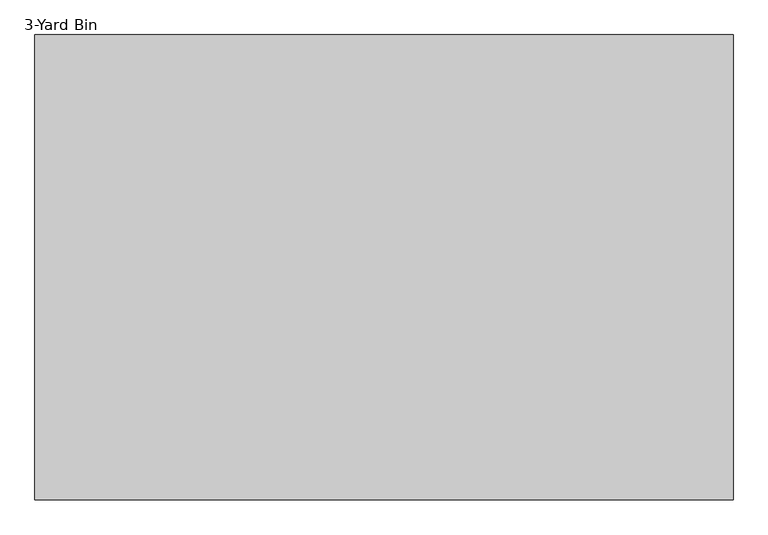
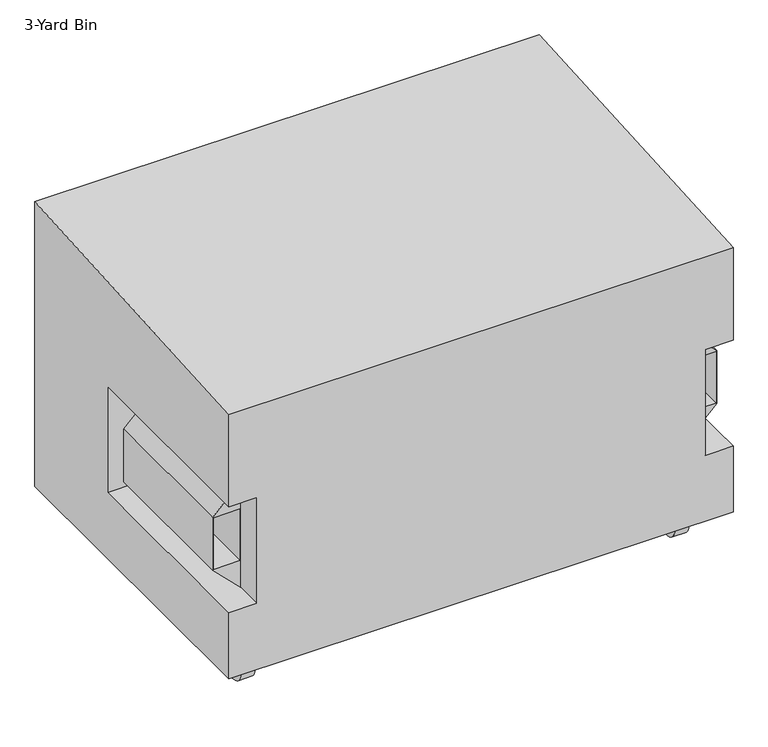
"""IFC4 building model written with IfcOpenShell, lengths in millimetres: proxy geometry, 323323 - Site Trash and Litter Receptacles - Dumpsters : 3-Yard Bin."""

import ifcopenshell
import ifcopenshell.guid

model = None  # the IFC model being written
_history = None  # IfcOwnerHistory: only IFC2X3 demands one
_inside = {}  # id of a spatial element -> (the spatial element, [elements in it])
_under = {}  # id of a project, library or spatial element -> (it, [spatial elements below it])
_declared = {}  # id of a project -> (the project, [libraries it declares])
_typed = {}  # id of a type object -> (the type object, [elements of that type])
_made_of = {}  # id of a material, layer set ... -> (it, [elements and type objects made of it])


def new_model(schema):
    """Start an empty IFC model of exactly this schema.

    Asked for "IFC4X3", IfcOpenShell would pick the latest addendum, in which some entities
    have other attributes; the version numbers below select the first issue.
    IFC2X3 requires an IfcOwnerHistory on every rooted entity: one is made here for all.
    """
    global model, _history
    if schema == "IFC4X3":
        model = ifcopenshell.file(schema_version=(4, 3, 0, 0))
    else:
        model = ifcopenshell.file(schema=schema)
    _inside.clear()
    _under.clear()
    _declared.clear()
    _typed.clear()
    _made_of.clear()
    _history = None
    if model.schema == "IFC2X3":
        org = make("IfcOrganization", Name="unknown")
        user = make(
            "IfcPersonAndOrganization",
            ThePerson=make("IfcPerson", FamilyName="unknown"),
            TheOrganization=org,
        )
        app = make(
            "IfcApplication",
            ApplicationDeveloper=org,
            Version="unknown",
            ApplicationFullName="unknown",
            ApplicationIdentifier="unknown",
        )
        _history = make(
            "IfcOwnerHistory",
            OwningUser=user,
            OwningApplication=app,
            ChangeAction="ADDED",
            CreationDate=0,
        )
    return model


def make(cls, **values):
    """One entity of the class cls with the attributes given. An attribute that is None is left unset."""
    return model.create_entity(
        cls, **{name: value for name, value in values.items() if value is not None}
    )


def rooted(cls, **values):
    """An entity with a GlobalId (a new one), such as an element, a storey or a relation."""
    return make(cls, GlobalId=ifcopenshell.guid.new(), OwnerHistory=_history, **values)


def si_unit(unit_type, name, prefix=None):
    """IfcSIUnit, for example si_unit("LENGTHUNIT", "METRE", prefix="MILLI")."""
    return make("IfcSIUnit", UnitType=unit_type, Prefix=prefix, Name=name)


def assignment(units):
    """IfcUnitAssignment: the units of a project."""
    return None if units is None else make("IfcUnitAssignment", Units=units)


def point(xyz):
    """IfcCartesianPoint."""
    return None if xyz is None else make("IfcCartesianPoint", Coordinates=xyz)


def direction(xyz):
    """IfcDirection."""
    return None if xyz is None else make("IfcDirection", DirectionRatios=xyz)


def frame(location, z_axis=None, x_axis=None):
    """IfcAxis2Placement3D, a coordinate frame: its origin and axes. An axis left out is left unset."""
    return make(
        "IfcAxis2Placement3D",
        Location=point(location),
        Axis=direction(z_axis),
        RefDirection=direction(x_axis),
    )


def frame_2d(location, x_axis=None):
    """IfcAxis2Placement2D, a coordinate frame in the plane: its origin and x axis."""
    return make(
        "IfcAxis2Placement2D", Location=point(location), RefDirection=direction(x_axis)
    )


def origin():
    """The frame at (0, 0, 0) with its axes left unset."""
    return frame((0.0, 0.0, 0.0))


def place(relative_to, where):
    """IfcLocalPlacement: puts the frame where relative to a parent placement (None: the world)."""
    return make(
        "IfcLocalPlacement", PlacementRelTo=relative_to, RelativePlacement=where
    )


def context(
    kind, dimensions, precision=None, world=None, true_north=None, identifier=None
):
    """IfcGeometricRepresentationContext, for example the 3D "Model" context."""
    return make(
        "IfcGeometricRepresentationContext",
        ContextIdentifier=identifier,
        ContextType=kind,
        CoordinateSpaceDimension=dimensions,
        Precision=precision,
        WorldCoordinateSystem=world,
        TrueNorth=true_north,
    )


def project(units=None, contexts=None):
    """IfcProject with its units and contexts."""
    return rooted(
        "IfcProject",
        Name="project",
        RepresentationContexts=contexts,
        UnitsInContext=assignment(units),
    )


def spatial(cls, under=None, at=None, **own):
    """A site, building, storey or space (cls), placed at a placement, below another one or the project."""
    s = rooted(cls, ObjectPlacement=at, **own)
    if under is not None:
        _under.setdefault(under.id(), (under, []))[1].append(s)
    return s


def circle_curve(where, radius):
    """IfcCircle in the frame where."""
    return make("IfcCircle", Position=where, Radius=radius)


def trimmed(basis, trim1, trim2, sense, master):
    """IfcTrimmedCurve: the piece of a basis curve between two trims."""
    return make(
        "IfcTrimmedCurve",
        BasisCurve=basis,
        Trim1=trim1,
        Trim2=trim2,
        SenseAgreement=sense,
        MasterRepresentation=master,
    )


def segment(curve, same_sense, transition):
    """IfcCompositeCurveSegment."""
    return make(
        "IfcCompositeCurveSegment",
        Transition=transition,
        SameSense=same_sense,
        ParentCurve=curve,
    )


def composite_curve(segments, self_intersect=None):
    """IfcCompositeCurve: segments joined end to end."""
    return make("IfcCompositeCurve", Segments=segments, SelfIntersect=self_intersect)


def outline(outer, holes=None, kind="AREA"):
    """IfcArbitraryClosedProfileDef: a profile drawn as a closed curve; with holes, ...WithVoids."""
    if holes is None:
        return make("IfcArbitraryClosedProfileDef", ProfileType=kind, OuterCurve=outer)
    return make(
        "IfcArbitraryProfileDefWithVoids",
        ProfileType=kind,
        OuterCurve=outer,
        InnerCurves=holes,
    )


def extrude(swept, where, along, depth):
    """IfcExtrudedAreaSolid: the profile swept, set in the frame where, extruded along a direction by depth."""
    return make(
        "IfcExtrudedAreaSolid",
        SweptArea=swept,
        Position=where,
        ExtrudedDirection=direction(along),
        Depth=depth,
    )


def faces_of(points, faces, orient=None, outer=None):
    """IfcFace entities. A face is a list of loops; a loop is a list of indices into points, from 0.

    orient and outer hold one flag for each loop. By default every Orientation is true, the
    first loop of a face is its IfcFaceOuterBound and the others are IfcFaceBound.
    """
    made = []
    for i, loops in enumerate(faces):
        bounds = []
        for j, loop in enumerate(loops):
            is_outer = j == 0 if outer is None else outer[i][j]
            bounds.append(
                make(
                    "IfcFaceOuterBound" if is_outer else "IfcFaceBound",
                    Bound=make("IfcPolyLoop", Polygon=[points[k] for k in loop]),
                    Orientation=True if orient is None else orient[i][j],
                )
            )
        made.append(make("IfcFace", Bounds=bounds))
    return made


def faceted_brep(points, faces, orient=None, outer=None, voids=None):
    """IfcFacetedBrep: a solid bounded by flat faces; with voids (closed shells), ...WithVoids."""
    shared = [point(p) for p in points]
    hull = make("IfcClosedShell", CfsFaces=faces_of(shared, faces, orient, outer))
    if voids is None:
        return make("IfcFacetedBrep", Outer=hull)
    return make(
        "IfcFacetedBrepWithVoids",
        Outer=hull,
        Voids=[
            make(cls, CfsFaces=faces_of(shared, fs, o, b)) for cls, fs, o, b in voids
        ],
    )


def shape(context_of_items, identifier, shape_type, items):
    """IfcShapeRepresentation: the items that make up one representation, for example the "Body"."""
    return make(
        "IfcShapeRepresentation",
        ContextOfItems=context_of_items,
        RepresentationIdentifier=identifier,
        RepresentationType=shape_type,
        Items=items,
    )


def source(mapping_origin, context_of_items, identifier, shape_type, items):
    """IfcRepresentationMap: a shape defined once, which mapped items show again and again."""
    return make(
        "IfcRepresentationMap",
        MappingOrigin=mapping_origin,
        MappedRepresentation=shape(context_of_items, identifier, shape_type, items),
    )


def transform(
    local_origin,
    x_axis=None,
    y_axis=None,
    z_axis=None,
    scale=None,
    scale2=None,
    scale3=None,
    uniform=True,
):
    """IfcCartesianTransformationOperator3D, or its non-uniform kind. x_axis, y_axis, z_axis: its Axis1, 2, 3."""
    if uniform:
        return make(
            "IfcCartesianTransformationOperator3D",
            Axis1=direction(x_axis),
            Axis2=direction(y_axis),
            LocalOrigin=point(local_origin),
            Scale=scale,
            Axis3=direction(z_axis),
        )
    return make(
        "IfcCartesianTransformationOperator3DnonUniform",
        Axis1=direction(x_axis),
        Axis2=direction(y_axis),
        LocalOrigin=point(local_origin),
        Scale=scale,
        Axis3=direction(z_axis),
        Scale2=scale2,
        Scale3=scale3,
    )


def mapped(mapping_source, mapping_target):
    """IfcMappedItem: shows the shape of a source again, moved by a transform."""
    return make(
        "IfcMappedItem", MappingSource=mapping_source, MappingTarget=mapping_target
    )


def made_of(thing, what):
    """Note that an element or type object is made of a material, layer set ...; save() writes the relation."""
    if what is not None:
        _made_of.setdefault(what.id(), (what, []))[1].append(thing)
    return thing


def element(
    cls,
    number,
    at=None,
    inside=None,
    cuts=None,
    type_object=None,
    material=None,
    context=None,
    identifier="Body",
    shape_type=None,
    held_by="IfcProductDefinitionShape",
    body=None,
    shapes=None,
    **own,
):
    """One element of the class cls, such as IfcWall. Its Tag is "e" and its number.

    at: its placement. inside: the storey or other place that contains it. cuts: it is an
    opening in that element (IfcRelVoidsElement). A single representation is given by context,
    identifier, shape_type and body (its items); several are given by shapes. held_by: the class
    of the entity that holds the representations. save() writes the other relations.
    """
    e = rooted(cls, Tag="e%d" % number, ObjectPlacement=at, **own)
    if body is not None:
        shapes = [shape(context, identifier, shape_type, body)]
    if shapes is not None:
        e.Representation = make(held_by, Representations=shapes)
    if inside is not None:
        _inside.setdefault(inside.id(), (inside, []))[1].append(e)
    if cuts is not None:
        rooted(
            "IfcRelVoidsElement", RelatingBuildingElement=cuts, RelatedOpeningElement=e
        )
    if type_object is not None:
        _typed.setdefault(type_object.id(), (type_object, []))[1].append(e)
    return made_of(e, material)


def aggregate(whole, parts):
    """IfcRelAggregates: a whole, such as a stair, and the parts it consists of."""
    return rooted("IfcRelAggregates", RelatingObject=whole, RelatedObjects=parts)


def save(model, path):
    """Write the relations noted so far, then the file.

    IfcRelAggregates (storeys below a building ...), IfcRelContainedInSpatialStructure (elements
    in a storey), IfcRelDefinesByType, IfcRelAssociatesMaterial and IfcRelDeclares: one each for
    every whole, place, type object, material and project.
    """
    for whole, parts in _under.values():
        aggregate(whole, parts)
    for where, things in _inside.values():
        rooted(
            "IfcRelContainedInSpatialStructure",
            RelatedElements=things,
            RelatingStructure=where,
        )
    for kind, things in _typed.values():
        rooted("IfcRelDefinesByType", RelatedObjects=things, RelatingType=kind)
    for what, things in _made_of.values():
        rooted("IfcRelAssociatesMaterial", RelatedObjects=things, RelatingMaterial=what)
    for by, libraries in _declared.values():
        rooted("IfcRelDeclares", RelatingContext=by, RelatedDefinitions=libraries)
    model.write(path)


def proxy_3_yard_bin_d6c0c25e(model_context):
    return source(origin(), model_context, "Body", "SolidModel", [
        faceted_brep([(914.4, 609.6, 127.0), (914.4, 609.6, 1219.2), (914.4, -609.6, 1143.0), (914.4, -609.6, 787.4), (914.4, -508.0, 787.4), (914.4, 50.8, 787.4), (914.4, 152.4, 787.4), (914.4, 152.4, 381.0), (914.4, 50.8, 381.0), (914.4, -508.0, 381.0), (914.4, -609.6, 381.0), (914.4, -609.6, 127.0), (914.4, -508.0, 685.8), (914.4, -508.0, 482.6), (914.4, 50.8, 482.6), (914.4, 50.8, 685.8), (-914.4, 609.6, 127.0), (-914.4, -609.6, 127.0), (-914.4, -609.6, 381.0), (-914.4, -508.0, 381.0), (-914.4, 50.8, 381.0), (-914.4, 152.4, 381.0), (-914.4, 152.4, 787.4), (-914.4, 50.8, 787.4), (-914.4, -508.0, 787.4), (-914.4, -609.6, 787.4), (-914.4, -609.6, 1143.0), (-914.4, 609.6, 1219.2), (-914.4, -508.0, 482.6), (-914.4, -508.0, 685.8), (-914.4, 50.8, 685.8), (-914.4, 50.8, 482.6), (-812.8, -609.6, 787.4), (-812.8, -609.6, 381.0), (812.8, -609.6, 381.0), (812.8, -609.6, 787.4), (812.8, 152.4, 787.4), (812.8, 152.4, 381.0), (-812.8, 152.4, 787.4), (-812.8, 152.4, 381.0), (-812.8, 50.8, 787.4), (-812.8, -508.0, 787.4), (-812.8, -508.0, 381.0), (-812.8, 50.8, 381.0), (-911.225, -508.0, 485.775), (-815.975, -508.0, 485.775), (-815.975, 50.8, 485.775), (-911.225, 50.8, 485.775), (-815.975, -508.0, 682.625), (-815.975, 50.8, 682.625), (-911.225, -508.0, 682.625), (-911.225, 50.8, 682.625), (812.8, -508.0, 787.4), (812.8, 50.8, 787.4), (812.8, 50.8, 381.0), (812.8, -508.0, 381.0), (911.225, -508.0, 485.775), (911.225, -508.0, 682.625), (911.225, 50.8, 682.625), (911.225, 50.8, 485.775), (815.975, -508.0, 682.625), (815.975, 50.8, 682.625), (815.975, -508.0, 485.775), (815.975, 50.8, 485.775)], [[[0, 1, 2, 3, 4, 5, 6, 7, 8, 9, 10, 11]], [[12, 13, 14, 15]], [[16, 17, 18, 19, 20, 21, 22, 23, 24, 25, 26, 27]], [[28, 29, 30, 31]], [[1, 0, 16, 27]], [[2, 1, 27, 26]], [[2, 26, 25, 32, 33, 18, 17, 11, 10, 34, 35, 3]], [[0, 11, 17, 16]], [[6, 36, 37, 7]], [[38, 22, 21, 39]], [[22, 38, 40, 41, 32, 25, 24, 23]], [[29, 41, 40, 30]], [[42, 28, 31, 43]], [[39, 21, 20, 19, 18, 33, 42, 43]], [[44, 45, 46, 47]], [[45, 48, 49, 46]], [[48, 50, 51, 49]], [[50, 44, 47, 51]], [[52, 12, 15, 53]], [[36, 6, 5, 4, 3, 35, 52, 53]], [[7, 37, 54, 55, 34, 10, 9, 8]], [[13, 55, 54, 14]], [[56, 57, 58, 59]], [[57, 60, 61, 58]], [[60, 62, 63, 61]], [[62, 56, 59, 63]], [[41, 42, 33, 32]], [[42, 41, 29, 28], [45, 44, 50, 48]], [[55, 52, 35, 34]], [[52, 55, 13, 12], [57, 56, 62, 60]], [[43, 40, 38, 39]], [[40, 43, 31, 30], [47, 46, 49, 51]], [[37, 36, 53, 54]], [[54, 53, 15, 14], [59, 58, 61, 63]]]),
        extrude(outline(composite_curve([segment(trimmed(circle_curve(frame_2d((-457.2, 50.8)), 50.8), [point((-508.0, 50.8))], [point((-406.4, 50.8))], False, "CARTESIAN"), True, "CONTINUOUS"), segment(trimmed(circle_curve(frame_2d((-457.2, 50.8)), 50.8), [point((-406.4, 50.8))], [point((-508.0, 50.8))], False, "CARTESIAN"), True, "CONTINUOUS")], self_intersect=False)), frame((762.0, 0.0, 0.0), z_axis=(1.0, 0.0, 0.0), x_axis=(0.0, 1.0, 0.0)), (0.0, 0.0, 1.0), 50.8),
        extrude(outline(composite_curve([segment(trimmed(circle_curve(frame_2d((457.2, 50.8)), 50.8), [point((406.4, 50.8))], [point((508.0, 50.8))], False, "CARTESIAN"), True, "CONTINUOUS"), segment(trimmed(circle_curve(frame_2d((457.2, 50.8)), 50.8), [point((508.0, 50.8))], [point((406.4, 50.8))], False, "CARTESIAN"), True, "CONTINUOUS")], self_intersect=False)), frame((762.0, 0.0, 0.0), z_axis=(1.0, 0.0, 0.0), x_axis=(0.0, 1.0, 0.0)), (0.0, 0.0, 1.0), 50.8),
        extrude(outline(composite_curve([segment(trimmed(circle_curve(frame_2d((457.2, 50.8)), 50.8), [point((406.4, 50.8))], [point((508.0, 50.8))], False, "CARTESIAN"), True, "CONTINUOUS"), segment(trimmed(circle_curve(frame_2d((457.2, 50.8)), 50.8), [point((508.0, 50.8))], [point((406.4, 50.8))], False, "CARTESIAN"), True, "CONTINUOUS")], self_intersect=False)), frame((-812.8, 0.0, 0.0), z_axis=(1.0, 0.0, 0.0), x_axis=(0.0, 1.0, 0.0)), (0.0, 0.0, 1.0), 50.8),
        extrude(outline(composite_curve([segment(trimmed(circle_curve(frame_2d((-457.2, 50.8)), 50.8), [point((-508.0, 50.8))], [point((-406.4, 50.8))], False, "CARTESIAN"), True, "CONTINUOUS"), segment(trimmed(circle_curve(frame_2d((-457.2, 50.8)), 50.8), [point((-406.4, 50.8))], [point((-508.0, 50.8))], False, "CARTESIAN"), True, "CONTINUOUS")], self_intersect=False)), frame((-812.8, 0.0, 0.0), z_axis=(1.0, 0.0, 0.0), x_axis=(0.0, 1.0, 0.0)), (0.0, 0.0, 1.0), 50.8),
    ])


if __name__ == "__main__":
    model = new_model("IFC4")
    model_context = context("Model", 3, world=origin())
    ifc_project = project(units=[si_unit("LENGTHUNIT", "METRE", prefix="MILLI")], contexts=[model_context])
    site = spatial("IfcSite", under=ifc_project)
    building = spatial("IfcBuilding", under=site)
    placement = place(None, origin())
    proxy_3_yard_bin_shape = proxy_3_yard_bin_d6c0c25e(model_context)
    element("IfcBuildingElementProxy", 1, Name="323323 - Site Trash and Litter Receptacles - Dumpsters : 3-Yard Bin", ObjectType="323323 - Site Trash and Litter Receptacles - Dumpsters : 3-Yard Bin", at=placement, inside=building, context=model_context, shape_type="MappedRepresentation", body=[
        mapped(proxy_3_yard_bin_shape, transform((0.0, 0.0, 0.0), x_axis=(1.0, 0.0, 0.0), y_axis=(0.0, 1.0, 0.0), z_axis=(0.0, 0.0, 1.0))),
    ])
    save(model, "model.ifc")

# Revit data of these elements
# Type "323323 - Site Trash and Litter Receptacles - Dumpsters : 3-Yard Bin"
#   WIDTH = 6' - 0"
#   HEIGHT - REAR = 4' - 0"
#   HEIGHT - FRONT = 3' - 9"
#   DEPTH = 4' - 0"
#   Material = 3 YARD GREASE BIN
# Element 1 (IfcBuildingElementProxy, "323323 - Site Trash and Litter Receptacles - Dumpsters : 3-Yard Bin")
#   Materials on its faces: "3 YARD GREASE BIN"
# Materials
#   "3 YARD GREASE BIN": class "Unassigned", colour RGB 214 209 182, transparency 0, Comments = "Rendering appearance not upgraded ", Cost = 0
